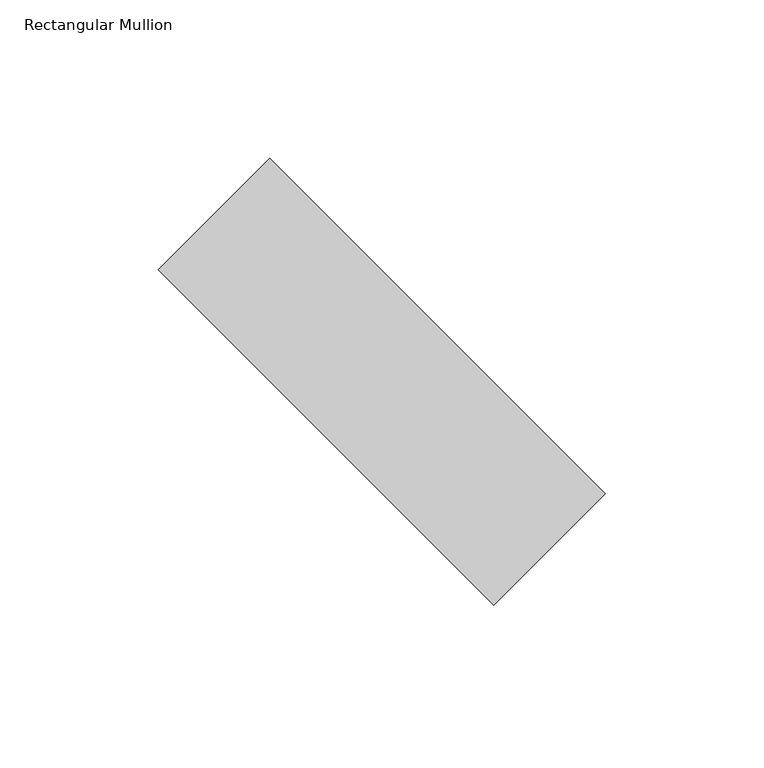
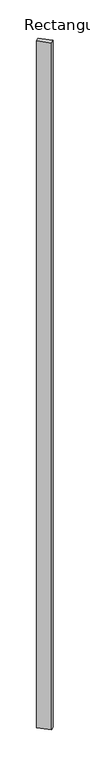
"""IFC4 building model written with IfcOpenShell, lengths in millimetres: member geometry, Rectangular Mullion : tilted mullions."""

from ifc_helpers import new_model, si_unit, frame, origin, place, context, project, spatial, polyline, outline, extrude, source, transform, mapped, element, save


def rectangular_mullion_0e496170(model_context):
    return source(origin(), model_context, "Body", "SweptSolid", [
        extrude(outline(polyline([(-35.3553391, 70.7106781), (70.7106781, -35.3553391), (35.3553391, -70.7106781), (-70.7106781, 35.3553391), (-35.3553391, 70.7106781)])), frame((0.0, 0.0, -8000.0002611), z_axis=(0.0, 0.0, 1.0), x_axis=(1.0, 0.0, 0.0)), (0.0, 0.0, 1.0), 8000.0002611),
    ])


if __name__ == "__main__":
    model = new_model("IFC4")
    model_context = context("Model", 3, world=origin())
    ifc_project = project(units=[si_unit("LENGTHUNIT", "METRE", prefix="MILLI")], contexts=[model_context])
    site = spatial("IfcSite", under=ifc_project)
    building = spatial("IfcBuilding", under=site)
    placement = place(None, origin())
    rectangular_mullion_shape = rectangular_mullion_0e496170(model_context)
    element("IfcMember", 1, ObjectType="Rectangular Mullion : tilted mullions", at=placement, inside=building, context=model_context, shape_type="MappedRepresentation", body=[
        mapped(rectangular_mullion_shape, transform((0.0, 0.0, 0.0), x_axis=(1.0, 0.0, 0.0), y_axis=(0.0, 1.0, 0.0), z_axis=(0.0, 0.0, 1.0))),
    ])
    save(model, "model.ifc")

# Revit data of these elements
# Type "Rectangular Mullion : tilted mullions"
#   built-in parameter 1007304 = 0.492126 (stored number, unit not read)
#   built-in parameter 1007301 = 0.082021 (stored number, unit not read)
#   built-in parameter 1007300 = 0.082021 (stored number, unit not read)
# Element 1 (IfcMember, "Rectangular Mullion : tilted mullions")
#   Materials on its faces: "Aluminum"
# Materials
#   "Aluminum": class "Metal", colour RGB 244 244 244, transparency 0, Description = "Aluminum 6061", Cost = 0
